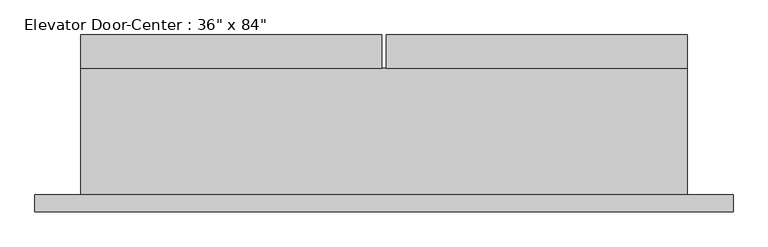
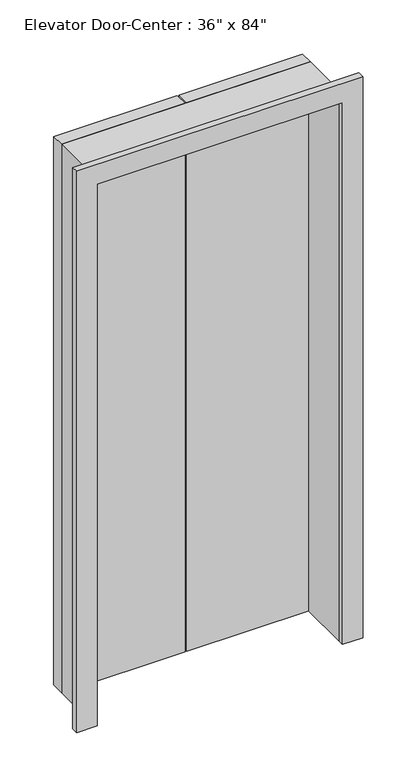
"""IFC4 building model written with IfcOpenShell, lengths in millimetres: proxy geometry."""

import ifcopenshell
import ifcopenshell.guid

model = None  # the IFC model being written
_history = None  # IfcOwnerHistory: only IFC2X3 demands one
_inside = {}  # id of a spatial element -> (the spatial element, [elements in it])
_under = {}  # id of a project, library or spatial element -> (it, [spatial elements below it])
_declared = {}  # id of a project -> (the project, [libraries it declares])
_typed = {}  # id of a type object -> (the type object, [elements of that type])
_made_of = {}  # id of a material, layer set ... -> (it, [elements and type objects made of it])


def new_model(schema):
    """Start an empty IFC model of exactly this schema.

    Asked for "IFC4X3", IfcOpenShell would pick the latest addendum, in which some entities
    have other attributes; the version numbers below select the first issue.
    IFC2X3 requires an IfcOwnerHistory on every rooted entity: one is made here for all.
    """
    global model, _history
    if schema == "IFC4X3":
        model = ifcopenshell.file(schema_version=(4, 3, 0, 0))
    else:
        model = ifcopenshell.file(schema=schema)
    _inside.clear()
    _under.clear()
    _declared.clear()
    _typed.clear()
    _made_of.clear()
    _history = None
    if model.schema == "IFC2X3":
        org = make("IfcOrganization", Name="unknown")
        user = make(
            "IfcPersonAndOrganization",
            ThePerson=make("IfcPerson", FamilyName="unknown"),
            TheOrganization=org,
        )
        app = make(
            "IfcApplication",
            ApplicationDeveloper=org,
            Version="unknown",
            ApplicationFullName="unknown",
            ApplicationIdentifier="unknown",
        )
        _history = make(
            "IfcOwnerHistory",
            OwningUser=user,
            OwningApplication=app,
            ChangeAction="ADDED",
            CreationDate=0,
        )
    return model


def make(cls, **values):
    """One entity of the class cls with the attributes given. An attribute that is None is left unset."""
    return model.create_entity(
        cls, **{name: value for name, value in values.items() if value is not None}
    )


def rooted(cls, **values):
    """An entity with a GlobalId (a new one), such as an element, a storey or a relation."""
    return make(cls, GlobalId=ifcopenshell.guid.new(), OwnerHistory=_history, **values)


def si_unit(unit_type, name, prefix=None):
    """IfcSIUnit, for example si_unit("LENGTHUNIT", "METRE", prefix="MILLI")."""
    return make("IfcSIUnit", UnitType=unit_type, Prefix=prefix, Name=name)


def assignment(units):
    """IfcUnitAssignment: the units of a project."""
    return None if units is None else make("IfcUnitAssignment", Units=units)


def point(xyz):
    """IfcCartesianPoint."""
    return None if xyz is None else make("IfcCartesianPoint", Coordinates=xyz)


def direction(xyz):
    """IfcDirection."""
    return None if xyz is None else make("IfcDirection", DirectionRatios=xyz)


def frame(location, z_axis=None, x_axis=None):
    """IfcAxis2Placement3D, a coordinate frame: its origin and axes. An axis left out is left unset."""
    return make(
        "IfcAxis2Placement3D",
        Location=point(location),
        Axis=direction(z_axis),
        RefDirection=direction(x_axis),
    )


def origin():
    """The frame at (0, 0, 0) with its axes left unset."""
    return frame((0.0, 0.0, 0.0))


def origin_with_axes():
    """The frame at (0, 0, 0) with the z axis (0, 0, 1) and the x axis (1, 0, 0) written out."""
    return frame((0.0, 0.0, 0.0), z_axis=(0.0, 0.0, 1.0), x_axis=(1.0, 0.0, 0.0))


def place(relative_to, where):
    """IfcLocalPlacement: puts the frame where relative to a parent placement (None: the world)."""
    return make(
        "IfcLocalPlacement", PlacementRelTo=relative_to, RelativePlacement=where
    )


def context(
    kind, dimensions, precision=None, world=None, true_north=None, identifier=None
):
    """IfcGeometricRepresentationContext, for example the 3D "Model" context."""
    return make(
        "IfcGeometricRepresentationContext",
        ContextIdentifier=identifier,
        ContextType=kind,
        CoordinateSpaceDimension=dimensions,
        Precision=precision,
        WorldCoordinateSystem=world,
        TrueNorth=true_north,
    )


def project(units=None, contexts=None):
    """IfcProject with its units and contexts."""
    return rooted(
        "IfcProject",
        Name="project",
        RepresentationContexts=contexts,
        UnitsInContext=assignment(units),
    )


def spatial(cls, under=None, at=None, **own):
    """A site, building, storey or space (cls), placed at a placement, below another one or the project."""
    s = rooted(cls, ObjectPlacement=at, **own)
    if under is not None:
        _under.setdefault(under.id(), (under, []))[1].append(s)
    return s


def polyline(points):
    """IfcPolyline through the points."""
    return make("IfcPolyline", Points=[point(p) for p in points])


def outline(outer, holes=None, kind="AREA"):
    """IfcArbitraryClosedProfileDef: a profile drawn as a closed curve; with holes, ...WithVoids."""
    if holes is None:
        return make("IfcArbitraryClosedProfileDef", ProfileType=kind, OuterCurve=outer)
    return make(
        "IfcArbitraryProfileDefWithVoids",
        ProfileType=kind,
        OuterCurve=outer,
        InnerCurves=holes,
    )


def extrude(swept, where, along, depth):
    """IfcExtrudedAreaSolid: the profile swept, set in the frame where, extruded along a direction by depth."""
    return make(
        "IfcExtrudedAreaSolid",
        SweptArea=swept,
        Position=where,
        ExtrudedDirection=direction(along),
        Depth=depth,
    )


def shape(context_of_items, identifier, shape_type, items):
    """IfcShapeRepresentation: the items that make up one representation, for example the "Body"."""
    return make(
        "IfcShapeRepresentation",
        ContextOfItems=context_of_items,
        RepresentationIdentifier=identifier,
        RepresentationType=shape_type,
        Items=items,
    )


def source(mapping_origin, context_of_items, identifier, shape_type, items):
    """IfcRepresentationMap: a shape defined once, which mapped items show again and again."""
    return make(
        "IfcRepresentationMap",
        MappingOrigin=mapping_origin,
        MappedRepresentation=shape(context_of_items, identifier, shape_type, items),
    )


def transform(
    local_origin,
    x_axis=None,
    y_axis=None,
    z_axis=None,
    scale=None,
    scale2=None,
    scale3=None,
    uniform=True,
):
    """IfcCartesianTransformationOperator3D, or its non-uniform kind. x_axis, y_axis, z_axis: its Axis1, 2, 3."""
    if uniform:
        return make(
            "IfcCartesianTransformationOperator3D",
            Axis1=direction(x_axis),
            Axis2=direction(y_axis),
            LocalOrigin=point(local_origin),
            Scale=scale,
            Axis3=direction(z_axis),
        )
    return make(
        "IfcCartesianTransformationOperator3DnonUniform",
        Axis1=direction(x_axis),
        Axis2=direction(y_axis),
        LocalOrigin=point(local_origin),
        Scale=scale,
        Axis3=direction(z_axis),
        Scale2=scale2,
        Scale3=scale3,
    )


def mapped(mapping_source, mapping_target):
    """IfcMappedItem: shows the shape of a source again, moved by a transform."""
    return make(
        "IfcMappedItem", MappingSource=mapping_source, MappingTarget=mapping_target
    )


def made_of(thing, what):
    """Note that an element or type object is made of a material, layer set ...; save() writes the relation."""
    if what is not None:
        _made_of.setdefault(what.id(), (what, []))[1].append(thing)
    return thing


def element(
    cls,
    number,
    at=None,
    inside=None,
    cuts=None,
    type_object=None,
    material=None,
    context=None,
    identifier="Body",
    shape_type=None,
    held_by="IfcProductDefinitionShape",
    body=None,
    shapes=None,
    **own,
):
    """One element of the class cls, such as IfcWall. Its Tag is "e" and its number.

    at: its placement. inside: the storey or other place that contains it. cuts: it is an
    opening in that element (IfcRelVoidsElement). A single representation is given by context,
    identifier, shape_type and body (its items); several are given by shapes. held_by: the class
    of the entity that holds the representations. save() writes the other relations.
    """
    e = rooted(cls, Tag="e%d" % number, ObjectPlacement=at, **own)
    if body is not None:
        shapes = [shape(context, identifier, shape_type, body)]
    if shapes is not None:
        e.Representation = make(held_by, Representations=shapes)
    if inside is not None:
        _inside.setdefault(inside.id(), (inside, []))[1].append(e)
    if cuts is not None:
        rooted(
            "IfcRelVoidsElement", RelatingBuildingElement=cuts, RelatedOpeningElement=e
        )
    if type_object is not None:
        _typed.setdefault(type_object.id(), (type_object, []))[1].append(e)
    return made_of(e, material)


def aggregate(whole, parts):
    """IfcRelAggregates: a whole, such as a stair, and the parts it consists of."""
    return rooted("IfcRelAggregates", RelatingObject=whole, RelatedObjects=parts)


def save(model, path):
    """Write the relations noted so far, then the file.

    IfcRelAggregates (storeys below a building ...), IfcRelContainedInSpatialStructure (elements
    in a storey), IfcRelDefinesByType, IfcRelAssociatesMaterial and IfcRelDeclares: one each for
    every whole, place, type object, material and project.
    """
    for whole, parts in _under.values():
        aggregate(whole, parts)
    for where, things in _inside.values():
        rooted(
            "IfcRelContainedInSpatialStructure",
            RelatedElements=things,
            RelatingStructure=where,
        )
    for kind, things in _typed.values():
        rooted("IfcRelDefinesByType", RelatedObjects=things, RelatingType=kind)
    for what, things in _made_of.values():
        rooted("IfcRelAssociatesMaterial", RelatedObjects=things, RelatingMaterial=what)
    for by, libraries in _declared.values():
        rooted("IfcRelDeclares", RelatingContext=by, RelatedDefinitions=libraries)
    model.write(path)


def proxy_71d7088b(model_context):
    return source(origin(), model_context, "Body", "SweptSolid", [
        extrude(outline(polyline([(-102.3106443, 96.8375), (-562.6856443, 96.8375), (-562.6856443, 147.6375), (-102.3106443, 147.6375), (-102.3106443, 96.8375)])), origin_with_axes(), (0.0, 0.0, 1.0), 2159.0),
        extrude(outline(polyline([(364.4143557, 96.8375), (-95.9606443, 96.8375), (-95.9606443, 147.6375), (364.4143557, 147.6375), (364.4143557, 96.8375)])), origin_with_axes(), (0.0, 0.0, 1.0), 2159.0),
        extrude(outline(polyline([(0.0, -562.6856443), (0.0, -556.3356443), (2133.6, -556.3356443), (2133.6, 358.0643557), (0.0, 358.0643557), (0.0, 364.4143557), (2159.0, 364.4143557), (2159.0, -562.6856443), (0.0, -562.6856443)])), frame((0.0, -96.8375, 0.0), z_axis=(0.0, 1.0, 0.0), x_axis=(0.0, 0.0, 1.0)), (0.0, 0.0, 1.0), 193.675),
        extrude(outline(polyline([(0.0, -632.5356443), (0.0, -556.3356443), (2133.6, -556.3356443), (2133.6, 358.0643557), (0.0, 358.0643557), (0.0, 434.2643557), (2209.8, 434.2643557), (2209.8, -632.5356443), (0.0, -632.5356443)])), frame((0.0, -122.2375, 0.0), z_axis=(0.0, 1.0, 0.0), x_axis=(0.0, 0.0, 1.0)), (0.0, 0.0, 1.0), 25.4),
    ])


if __name__ == "__main__":
    model = new_model("IFC4")
    model_context = context("Model", 3, world=origin())
    ifc_project = project(units=[si_unit("LENGTHUNIT", "METRE", prefix="MILLI")], contexts=[model_context])
    site = spatial("IfcSite", under=ifc_project)
    building = spatial("IfcBuilding", under=site)
    placement = place(None, origin())
    proxy_shape = proxy_71d7088b(model_context)
    element("IfcBuildingElementProxy", 1, Name="Elevator Door-Center : 36\" x 84\"", ObjectType="Elevator Door-Center : 36\" x 84\"", at=placement, inside=building, context=model_context, shape_type="MappedRepresentation", body=[
        mapped(proxy_shape, transform((0.0, 0.0, 0.0), x_axis=(1.0, 0.0, 0.0), y_axis=(0.0, 1.0, 0.0), z_axis=(0.0, 0.0, 1.0))),
    ])
    save(model, "model.ifc")

# Revit data of these elements
# Type "Elevator Door-Center : 36\" x 84\""
#   Assembly Code = "D1010"
#   Door Height = 7' - 0"
#   Door Width = 3' - 0"
#   Trim Projection = 0' - 1"
#   Trim Width = 0' - 3"
#   Door Finish = Elevator Door
#   Frame Finish = Door - Frame
#   Default Elevation = 0
# Element 1 (IfcBuildingElementProxy, "Elevator Door-Center : 36\" x 84\"")
#   Materials on its faces: "Door - Frame", "Elevator Door"
# Materials
#   "Elevator Door": class "Metal", colour RGB 57 57 57, transparency 0
#   "Door - Frame": class "Miscellaneous", colour RGB 118 70 51, transparency 0, Cost = 0
